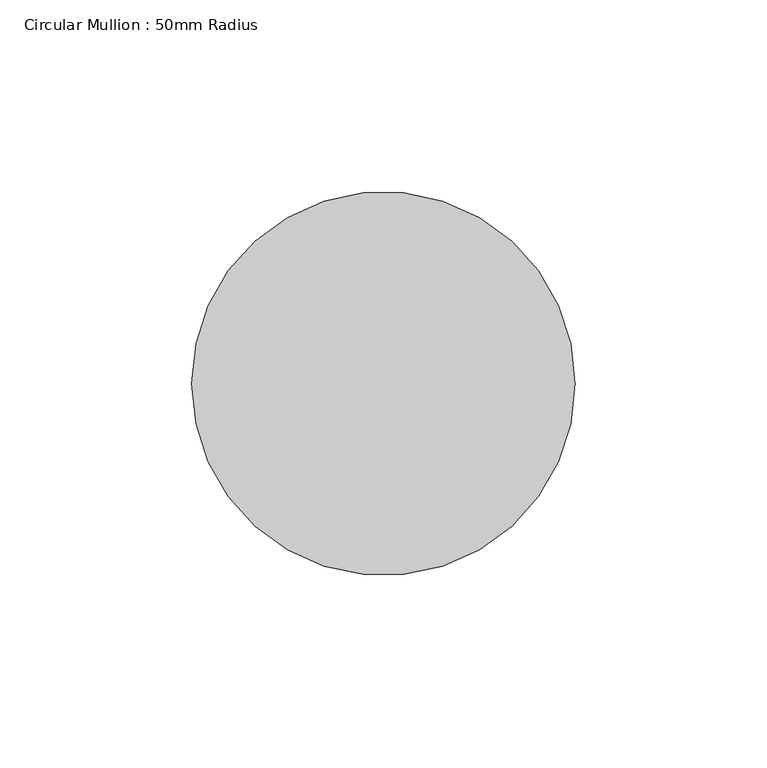
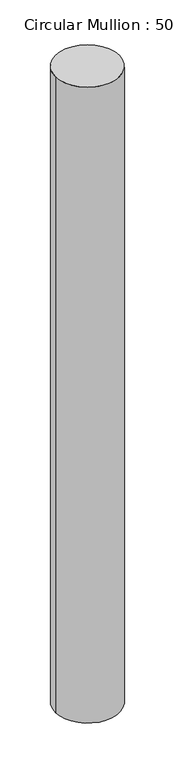
"""IFC4 building model written with IfcOpenShell, lengths in millimetres: member geometry, Circular Mullion : 50mm Radius."""

from ifc_helpers import new_model, si_unit, point, frame, origin, origin_2d, place, context, project, spatial, circle_curve, trimmed, segment, composite_curve, outline, extrude, source, transform, mapped, element, save


def circular_mullion_50mm_radius_304b95db(model_context):
    return source(origin(), model_context, "Body", "SweptSolid", [
        extrude(outline(composite_curve([segment(trimmed(circle_curve(origin_2d(), 50.0), [point((50.0, 0.0))], [point((-50.0, 0.0))], False, "CARTESIAN"), True, "CONTINUOUS"), segment(trimmed(circle_curve(origin_2d(), 50.0), [point((-50.0, 0.0))], [point((50.0, 0.0))], False, "CARTESIAN"), True, "CONTINUOUS")], self_intersect=False)), frame((0.0, 0.0, -1047.619804), z_axis=(0.0, 0.0, 1.0), x_axis=(1.0, 0.0, 0.0)), (0.0, 0.0, 1.0), 1047.619804),
    ])


if __name__ == "__main__":
    model = new_model("IFC4")
    model_context = context("Model", 3, world=origin())
    ifc_project = project(units=[si_unit("LENGTHUNIT", "METRE", prefix="MILLI")], contexts=[model_context])
    site = spatial("IfcSite", under=ifc_project)
    building = spatial("IfcBuilding", under=site)
    placement = place(None, origin())
    circular_mullion_50mm_radius_shape = circular_mullion_50mm_radius_304b95db(model_context)
    element("IfcMember", 1, ObjectType="Circular Mullion : 50mm Radius", at=placement, inside=building, context=model_context, shape_type="MappedRepresentation", body=[
        mapped(circular_mullion_50mm_radius_shape, transform((0.0, 0.0, 0.0), x_axis=(1.0, 0.0, 0.0), y_axis=(0.0, 1.0, 0.0), z_axis=(0.0, 0.0, 1.0))),
    ])
    save(model, "model.ifc")

# Revit data of these elements
# Type "Circular Mullion : 50mm Radius"
#   built-in parameter 1007350 = 0.164042 (stored number, unit not read)
# Element 1 (IfcMember, "Circular Mullion : 50mm Radius")
#   Materials on its faces: "Aluminium"
# Materials
#   "Aluminium": class "Metal", colour RGB 247 247 247, transparency 0, Description = "Aluminium 6061", Cost = 0
